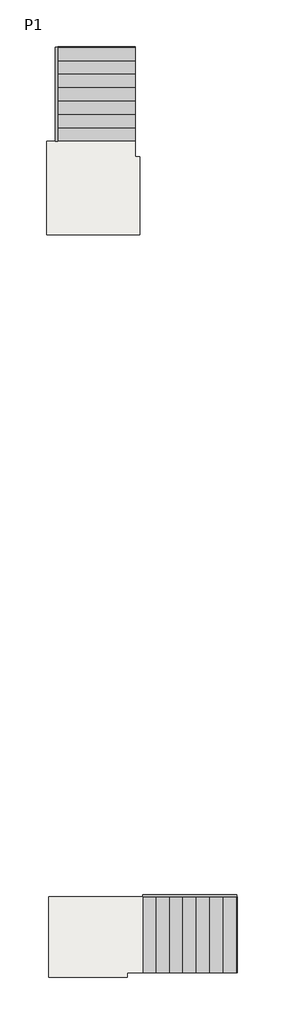
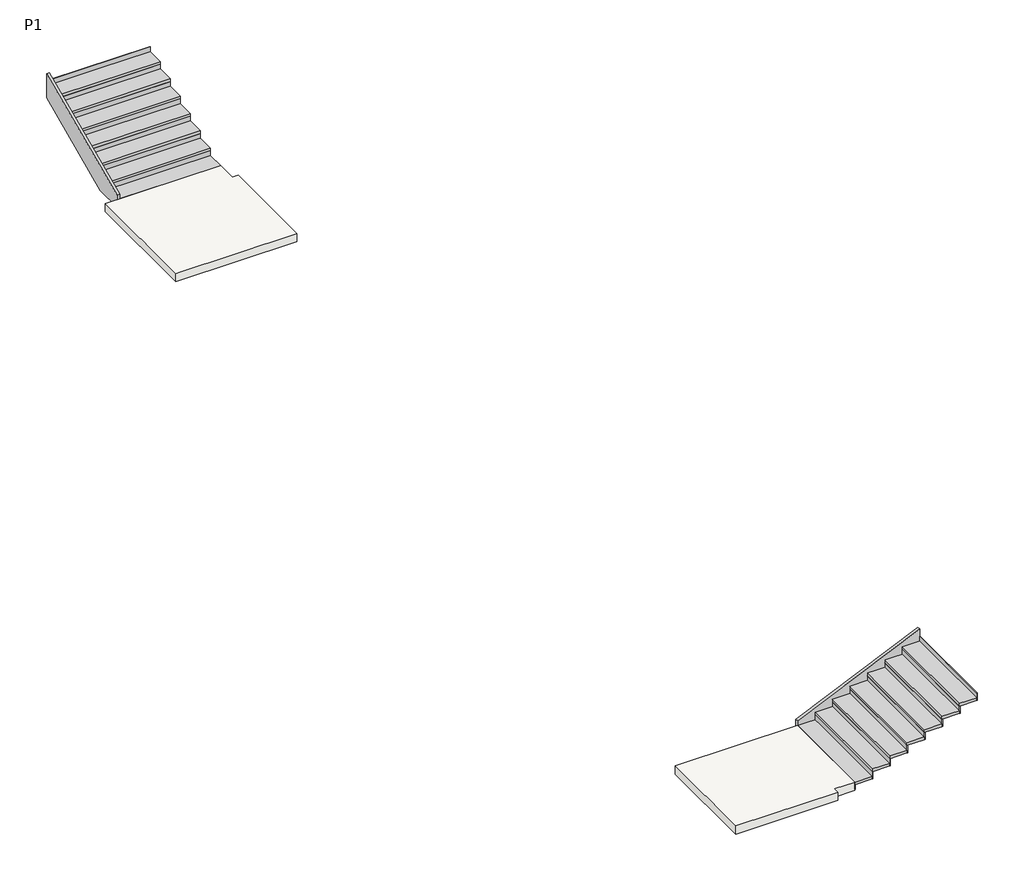
# One storey: 2 members, 2 slabs, 2 stair flights.
"""IFC4 building model written with IfcOpenShell, lengths in millimetres."""

import ifcopenshell
import ifcopenshell.guid

model = None  # the IFC model being written
_history = None  # IfcOwnerHistory: only IFC2X3 demands one
_inside = {}  # id of a spatial element -> (the spatial element, [elements in it])
_under = {}  # id of a project, library or spatial element -> (it, [spatial elements below it])
_declared = {}  # id of a project -> (the project, [libraries it declares])
_typed = {}  # id of a type object -> (the type object, [elements of that type])
_made_of = {}  # id of a material, layer set ... -> (it, [elements and type objects made of it])


def new_model(schema):
    """Start an empty IFC model of exactly this schema.

    Asked for "IFC4X3", IfcOpenShell would pick the latest addendum, in which some entities
    have other attributes; the version numbers below select the first issue.
    IFC2X3 requires an IfcOwnerHistory on every rooted entity: one is made here for all.
    """
    global model, _history
    if schema == "IFC4X3":
        model = ifcopenshell.file(schema_version=(4, 3, 0, 0))
    else:
        model = ifcopenshell.file(schema=schema)
    _inside.clear()
    _under.clear()
    _declared.clear()
    _typed.clear()
    _made_of.clear()
    _history = None
    if model.schema == "IFC2X3":
        org = make("IfcOrganization", Name="unknown")
        user = make(
            "IfcPersonAndOrganization",
            ThePerson=make("IfcPerson", FamilyName="unknown"),
            TheOrganization=org,
        )
        app = make(
            "IfcApplication",
            ApplicationDeveloper=org,
            Version="unknown",
            ApplicationFullName="unknown",
            ApplicationIdentifier="unknown",
        )
        _history = make(
            "IfcOwnerHistory",
            OwningUser=user,
            OwningApplication=app,
            ChangeAction="ADDED",
            CreationDate=0,
        )
    return model


def make(cls, **values):
    """One entity of the class cls with the attributes given. An attribute that is None is left unset."""
    return model.create_entity(
        cls, **{name: value for name, value in values.items() if value is not None}
    )


def rooted(cls, **values):
    """An entity with a GlobalId (a new one), such as an element, a storey or a relation."""
    return make(cls, GlobalId=ifcopenshell.guid.new(), OwnerHistory=_history, **values)


def si_unit(unit_type, name, prefix=None):
    """IfcSIUnit, for example si_unit("LENGTHUNIT", "METRE", prefix="MILLI")."""
    return make("IfcSIUnit", UnitType=unit_type, Prefix=prefix, Name=name)


def assignment(units):
    """IfcUnitAssignment: the units of a project."""
    return None if units is None else make("IfcUnitAssignment", Units=units)


def point(xyz):
    """IfcCartesianPoint."""
    return None if xyz is None else make("IfcCartesianPoint", Coordinates=xyz)


def direction(xyz):
    """IfcDirection."""
    return None if xyz is None else make("IfcDirection", DirectionRatios=xyz)


def frame(location, z_axis=None, x_axis=None):
    """IfcAxis2Placement3D, a coordinate frame: its origin and axes. An axis left out is left unset."""
    return make(
        "IfcAxis2Placement3D",
        Location=point(location),
        Axis=direction(z_axis),
        RefDirection=direction(x_axis),
    )


def origin():
    """The frame at (0, 0, 0) with its axes left unset."""
    return frame((0.0, 0.0, 0.0))


def place(relative_to, where):
    """IfcLocalPlacement: puts the frame where relative to a parent placement (None: the world)."""
    return make(
        "IfcLocalPlacement", PlacementRelTo=relative_to, RelativePlacement=where
    )


def context(
    kind, dimensions, precision=None, world=None, true_north=None, identifier=None
):
    """IfcGeometricRepresentationContext, for example the 3D "Model" context."""
    return make(
        "IfcGeometricRepresentationContext",
        ContextIdentifier=identifier,
        ContextType=kind,
        CoordinateSpaceDimension=dimensions,
        Precision=precision,
        WorldCoordinateSystem=world,
        TrueNorth=true_north,
    )


def project(units=None, contexts=None):
    """IfcProject with its units and contexts."""
    return rooted(
        "IfcProject",
        Name="project",
        RepresentationContexts=contexts,
        UnitsInContext=assignment(units),
    )


def spatial(cls, under=None, at=None, **own):
    """A site, building, storey or space (cls), placed at a placement, below another one or the project."""
    s = rooted(cls, ObjectPlacement=at, **own)
    if under is not None:
        _under.setdefault(under.id(), (under, []))[1].append(s)
    return s


def polyline(points):
    """IfcPolyline through the points."""
    return make("IfcPolyline", Points=[point(p) for p in points])


def outline(outer, holes=None, kind="AREA"):
    """IfcArbitraryClosedProfileDef: a profile drawn as a closed curve; with holes, ...WithVoids."""
    if holes is None:
        return make("IfcArbitraryClosedProfileDef", ProfileType=kind, OuterCurve=outer)
    return make(
        "IfcArbitraryProfileDefWithVoids",
        ProfileType=kind,
        OuterCurve=outer,
        InnerCurves=holes,
    )


def extrude(swept, where, along, depth):
    """IfcExtrudedAreaSolid: the profile swept, set in the frame where, extruded along a direction by depth."""
    return make(
        "IfcExtrudedAreaSolid",
        SweptArea=swept,
        Position=where,
        ExtrudedDirection=direction(along),
        Depth=depth,
    )


def shape(context_of_items, identifier, shape_type, items):
    """IfcShapeRepresentation: the items that make up one representation, for example the "Body"."""
    return make(
        "IfcShapeRepresentation",
        ContextOfItems=context_of_items,
        RepresentationIdentifier=identifier,
        RepresentationType=shape_type,
        Items=items,
    )


def source(mapping_origin, context_of_items, identifier, shape_type, items):
    """IfcRepresentationMap: a shape defined once, which mapped items show again and again."""
    return make(
        "IfcRepresentationMap",
        MappingOrigin=mapping_origin,
        MappedRepresentation=shape(context_of_items, identifier, shape_type, items),
    )


def transform(
    local_origin,
    x_axis=None,
    y_axis=None,
    z_axis=None,
    scale=None,
    scale2=None,
    scale3=None,
    uniform=True,
):
    """IfcCartesianTransformationOperator3D, or its non-uniform kind. x_axis, y_axis, z_axis: its Axis1, 2, 3."""
    if uniform:
        return make(
            "IfcCartesianTransformationOperator3D",
            Axis1=direction(x_axis),
            Axis2=direction(y_axis),
            LocalOrigin=point(local_origin),
            Scale=scale,
            Axis3=direction(z_axis),
        )
    return make(
        "IfcCartesianTransformationOperator3DnonUniform",
        Axis1=direction(x_axis),
        Axis2=direction(y_axis),
        LocalOrigin=point(local_origin),
        Scale=scale,
        Axis3=direction(z_axis),
        Scale2=scale2,
        Scale3=scale3,
    )


def mapped(mapping_source, mapping_target):
    """IfcMappedItem: shows the shape of a source again, moved by a transform."""
    return make(
        "IfcMappedItem", MappingSource=mapping_source, MappingTarget=mapping_target
    )


def made_of(thing, what):
    """Note that an element or type object is made of a material, layer set ...; save() writes the relation."""
    if what is not None:
        _made_of.setdefault(what.id(), (what, []))[1].append(thing)
    return thing


def element(
    cls,
    number,
    at=None,
    inside=None,
    cuts=None,
    type_object=None,
    material=None,
    context=None,
    identifier="Body",
    shape_type=None,
    held_by="IfcProductDefinitionShape",
    body=None,
    shapes=None,
    **own,
):
    """One element of the class cls, such as IfcWall. Its Tag is "e" and its number.

    at: its placement. inside: the storey or other place that contains it. cuts: it is an
    opening in that element (IfcRelVoidsElement). A single representation is given by context,
    identifier, shape_type and body (its items); several are given by shapes. held_by: the class
    of the entity that holds the representations. save() writes the other relations.
    """
    e = rooted(cls, Tag="e%d" % number, ObjectPlacement=at, **own)
    if body is not None:
        shapes = [shape(context, identifier, shape_type, body)]
    if shapes is not None:
        e.Representation = make(held_by, Representations=shapes)
    if inside is not None:
        _inside.setdefault(inside.id(), (inside, []))[1].append(e)
    if cuts is not None:
        rooted(
            "IfcRelVoidsElement", RelatingBuildingElement=cuts, RelatedOpeningElement=e
        )
    if type_object is not None:
        _typed.setdefault(type_object.id(), (type_object, []))[1].append(e)
    return made_of(e, material)


def aggregate(whole, parts):
    """IfcRelAggregates: a whole, such as a stair, and the parts it consists of."""
    return rooted("IfcRelAggregates", RelatingObject=whole, RelatedObjects=parts)


def save(model, path):
    """Write the relations noted so far, then the file.

    IfcRelAggregates (storeys below a building ...), IfcRelContainedInSpatialStructure (elements
    in a storey), IfcRelDefinesByType, IfcRelAssociatesMaterial and IfcRelDeclares: one each for
    every whole, place, type object, material and project.
    """
    for whole, parts in _under.values():
        aggregate(whole, parts)
    for where, things in _inside.values():
        rooted(
            "IfcRelContainedInSpatialStructure",
            RelatedElements=things,
            RelatingStructure=where,
        )
    for kind, things in _typed.values():
        rooted("IfcRelDefinesByType", RelatedObjects=things, RelatingType=kind)
    for what, things in _made_of.values():
        rooted("IfcRelAssociatesMaterial", RelatedObjects=things, RelatingMaterial=what)
    for by, libraries in _declared.values():
        rooted("IfcRelDeclares", RelatingContext=by, RelatedDefinitions=libraries)
    model.write(path)


def stair_flight_50mm_tread_13mm_riser_0aac887c(model_context):
    return source(origin(), model_context, "Body", "SweptSolid", [
        extrude(outline(polyline([(-15644.418089, 13093.1768963), (-15644.418089, 13080.6768963), (-17374.418089, 13080.6768963), (-17374.418089, 13093.1768963), (-15644.418089, 13093.1768963)])), frame((0.0, 0.0, -2133.3333333), z_axis=(0.0, 0.0, 1.0), x_axis=(1.0, 0.0, 0.0)), (0.0, 0.0, 1.0), 83.3333333),
        extrude(outline(polyline([(-17374.418089, 13380.6768963), (-15644.418089, 13380.6768963), (-15644.418089, 13080.6768963), (-17374.418089, 13080.6768963), (-17374.418089, 13380.6768963)])), frame((0.0, 0.0, -2050.0), z_axis=(0.0, 0.0, 1.0), x_axis=(1.0, 0.0, 0.0)), (0.0, 0.0, 1.0), 50.0),
        extrude(outline(polyline([(-15644.418089, 13393.1768963), (-15644.418089, 13380.6768963), (-17374.418089, 13380.6768963), (-17374.418089, 13393.1768963), (-15644.418089, 13393.1768963)])), frame((0.0, 0.0, -2050.0), z_axis=(0.0, 0.0, 1.0), x_axis=(1.0, 0.0, 0.0)), (0.0, 0.0, 1.0), 133.3333333),
        extrude(outline(polyline([(-17374.418089, 13680.6768963), (-15644.418089, 13680.6768963), (-15644.418089, 13380.6768963), (-17374.418089, 13380.6768963), (-17374.418089, 13680.6768963)])), frame((0.0, 0.0, -1916.6666667), z_axis=(0.0, 0.0, 1.0), x_axis=(1.0, 0.0, 0.0)), (0.0, 0.0, 1.0), 50.0),
        extrude(outline(polyline([(-15644.418089, 13693.1768963), (-15644.418089, 13680.6768963), (-17374.418089, 13680.6768963), (-17374.418089, 13693.1768963), (-15644.418089, 13693.1768963)])), frame((0.0, 0.0, -1916.6666667), z_axis=(0.0, 0.0, 1.0), x_axis=(1.0, 0.0, 0.0)), (0.0, 0.0, 1.0), 133.3333333),
        extrude(outline(polyline([(-17374.418089, 13980.6768963), (-15644.418089, 13980.6768963), (-15644.418089, 13680.6768963), (-17374.418089, 13680.6768963), (-17374.418089, 13980.6768963)])), frame((0.0, 0.0, -1783.3333333), z_axis=(0.0, 0.0, 1.0), x_axis=(1.0, 0.0, 0.0)), (0.0, 0.0, 1.0), 50.0),
        extrude(outline(polyline([(-15644.418089, 13993.1768963), (-15644.418089, 13980.6768963), (-17374.418089, 13980.6768963), (-17374.418089, 13993.1768963), (-15644.418089, 13993.1768963)])), frame((0.0, 0.0, -1783.3333333), z_axis=(0.0, 0.0, 1.0), x_axis=(1.0, 0.0, 0.0)), (0.0, 0.0, 1.0), 133.3333333),
        extrude(outline(polyline([(-17374.418089, 14280.6768963), (-15644.418089, 14280.6768963), (-15644.418089, 13980.6768963), (-17374.418089, 13980.6768963), (-17374.418089, 14280.6768963)])), frame((0.0, 0.0, -1650.0), z_axis=(0.0, 0.0, 1.0), x_axis=(1.0, 0.0, 0.0)), (0.0, 0.0, 1.0), 50.0),
        extrude(outline(polyline([(-15644.418089, 14293.1768963), (-15644.418089, 14280.6768963), (-17374.418089, 14280.6768963), (-17374.418089, 14293.1768963), (-15644.418089, 14293.1768963)])), frame((0.0, 0.0, -1650.0), z_axis=(0.0, 0.0, 1.0), x_axis=(1.0, 0.0, 0.0)), (0.0, 0.0, 1.0), 133.3333333),
        extrude(outline(polyline([(-17374.418089, 14580.6768963), (-15644.418089, 14580.6768963), (-15644.418089, 14280.6768963), (-17374.418089, 14280.6768963), (-17374.418089, 14580.6768963)])), frame((0.0, 0.0, -1516.6666667), z_axis=(0.0, 0.0, 1.0), x_axis=(1.0, 0.0, 0.0)), (0.0, 0.0, 1.0), 50.0),
        extrude(outline(polyline([(-15644.418089, 14593.1768963), (-15644.418089, 14580.6768963), (-17374.418089, 14580.6768963), (-17374.418089, 14593.1768963), (-15644.418089, 14593.1768963)])), frame((0.0, 0.0, -1516.6666667), z_axis=(0.0, 0.0, 1.0), x_axis=(1.0, 0.0, 0.0)), (0.0, 0.0, 1.0), 133.3333333),
        extrude(outline(polyline([(-17374.418089, 14880.6768963), (-15644.418089, 14880.6768963), (-15644.418089, 14580.6768963), (-17374.418089, 14580.6768963), (-17374.418089, 14880.6768963)])), frame((0.0, 0.0, -1383.3333333), z_axis=(0.0, 0.0, 1.0), x_axis=(1.0, 0.0, 0.0)), (0.0, 0.0, 1.0), 50.0),
        extrude(outline(polyline([(-15644.418089, 14893.1768963), (-15644.418089, 14880.6768963), (-17374.418089, 14880.6768963), (-17374.418089, 14893.1768963), (-15644.418089, 14893.1768963)])), frame((0.0, 0.0, -1383.3333333), z_axis=(0.0, 0.0, 1.0), x_axis=(1.0, 0.0, 0.0)), (0.0, 0.0, 1.0), 133.3333333),
        extrude(outline(polyline([(-15644.418089, 15193.1768963), (-15644.418089, 15180.6768963), (-17374.418089, 15180.6768963), (-17374.418089, 15193.1768963), (-15644.418089, 15193.1768963)])), frame((0.0, 0.0, -1250.0), z_axis=(0.0, 0.0, 1.0), x_axis=(1.0, 0.0, 0.0)), (0.0, 0.0, 1.0), 133.3333333),
        extrude(outline(polyline([(-17374.418089, 15180.6768963), (-15644.418089, 15180.6768963), (-15644.418089, 14880.6768963), (-17374.418089, 14880.6768963), (-17374.418089, 15180.6768963)])), frame((0.0, 0.0, -1250.0), z_axis=(0.0, 0.0, 1.0), x_axis=(1.0, 0.0, 0.0)), (0.0, 0.0, 1.0), 50.0),
    ])


def stair_flight_50mm_tread_13mm_riser_cbb1d095(model_context):
    return source(origin(), model_context, "Body", "SweptSolid", [
        extrude(outline(polyline([(-15462.7814495, -5518.0731037), (-15475.2814495, -5518.0731037), (-15475.2814495, -3818.0731037), (-15462.7814495, -3818.0731037), (-15462.7814495, -5518.0731037)])), frame((0.0, 0.0, -2133.3333333), z_axis=(0.0, 0.0, 1.0), x_axis=(1.0, 0.0, 0.0)), (0.0, 0.0, 1.0), 83.3333333),
        extrude(outline(polyline([(-15175.2814495, -3818.0731037), (-15175.2814495, -5518.0731037), (-15475.2814495, -5518.0731037), (-15475.2814495, -3818.0731037), (-15175.2814495, -3818.0731037)])), frame((0.0, 0.0, -2050.0), z_axis=(0.0, 0.0, 1.0), x_axis=(1.0, 0.0, 0.0)), (0.0, 0.0, 1.0), 50.0),
        extrude(outline(polyline([(-15162.7814495, -5518.0731037), (-15175.2814495, -5518.0731037), (-15175.2814495, -3818.0731037), (-15162.7814495, -3818.0731037), (-15162.7814495, -5518.0731037)])), frame((0.0, 0.0, -2050.0), z_axis=(0.0, 0.0, 1.0), x_axis=(1.0, 0.0, 0.0)), (0.0, 0.0, 1.0), 133.3333333),
        extrude(outline(polyline([(-14875.2814495, -3818.0731037), (-14875.2814495, -5518.0731037), (-15175.2814495, -5518.0731037), (-15175.2814495, -3818.0731037), (-14875.2814495, -3818.0731037)])), frame((0.0, 0.0, -1916.6666667), z_axis=(0.0, 0.0, 1.0), x_axis=(1.0, 0.0, 0.0)), (0.0, 0.0, 1.0), 50.0),
        extrude(outline(polyline([(-14862.7814495, -5518.0731037), (-14875.2814495, -5518.0731037), (-14875.2814495, -3818.0731037), (-14862.7814495, -3818.0731037), (-14862.7814495, -5518.0731037)])), frame((0.0, 0.0, -1916.6666667), z_axis=(0.0, 0.0, 1.0), x_axis=(1.0, 0.0, 0.0)), (0.0, 0.0, 1.0), 133.3333333),
        extrude(outline(polyline([(-14575.2814495, -3818.0731037), (-14575.2814495, -5518.0731037), (-14875.2814495, -5518.0731037), (-14875.2814495, -3818.0731037), (-14575.2814495, -3818.0731037)])), frame((0.0, 0.0, -1783.3333333), z_axis=(0.0, 0.0, 1.0), x_axis=(1.0, 0.0, 0.0)), (0.0, 0.0, 1.0), 50.0),
        extrude(outline(polyline([(-14562.7814495, -5518.0731037), (-14575.2814495, -5518.0731037), (-14575.2814495, -3818.0731037), (-14562.7814495, -3818.0731037), (-14562.7814495, -5518.0731037)])), frame((0.0, 0.0, -1783.3333333), z_axis=(0.0, 0.0, 1.0), x_axis=(1.0, 0.0, 0.0)), (0.0, 0.0, 1.0), 133.3333333),
        extrude(outline(polyline([(-14275.2814495, -3818.0731037), (-14275.2814495, -5518.0731037), (-14575.2814495, -5518.0731037), (-14575.2814495, -3818.0731037), (-14275.2814495, -3818.0731037)])), frame((0.0, 0.0, -1650.0), z_axis=(0.0, 0.0, 1.0), x_axis=(1.0, 0.0, 0.0)), (0.0, 0.0, 1.0), 50.0),
        extrude(outline(polyline([(-14262.7814495, -5518.0731037), (-14275.2814495, -5518.0731037), (-14275.2814495, -3818.0731037), (-14262.7814495, -3818.0731037), (-14262.7814495, -5518.0731037)])), frame((0.0, 0.0, -1650.0), z_axis=(0.0, 0.0, 1.0), x_axis=(1.0, 0.0, 0.0)), (0.0, 0.0, 1.0), 133.3333333),
        extrude(outline(polyline([(-13975.2814495, -3818.0731037), (-13975.2814495, -5518.0731037), (-14275.2814495, -5518.0731037), (-14275.2814495, -3818.0731037), (-13975.2814495, -3818.0731037)])), frame((0.0, 0.0, -1516.6666667), z_axis=(0.0, 0.0, 1.0), x_axis=(1.0, 0.0, 0.0)), (0.0, 0.0, 1.0), 50.0),
        extrude(outline(polyline([(-13962.7814495, -5518.0731037), (-13975.2814495, -5518.0731037), (-13975.2814495, -3818.0731037), (-13962.7814495, -3818.0731037), (-13962.7814495, -5518.0731037)])), frame((0.0, 0.0, -1516.6666667), z_axis=(0.0, 0.0, 1.0), x_axis=(1.0, 0.0, 0.0)), (0.0, 0.0, 1.0), 133.3333333),
        extrude(outline(polyline([(-13675.2814495, -3818.0731037), (-13675.2814495, -5518.0731037), (-13975.2814495, -5518.0731037), (-13975.2814495, -3818.0731037), (-13675.2814495, -3818.0731037)])), frame((0.0, 0.0, -1383.3333333), z_axis=(0.0, 0.0, 1.0), x_axis=(1.0, 0.0, 0.0)), (0.0, 0.0, 1.0), 50.0),
        extrude(outline(polyline([(-13662.7814495, -5518.0731037), (-13675.2814495, -5518.0731037), (-13675.2814495, -3818.0731037), (-13662.7814495, -3818.0731037), (-13662.7814495, -5518.0731037)])), frame((0.0, 0.0, -1383.3333333), z_axis=(0.0, 0.0, 1.0), x_axis=(1.0, 0.0, 0.0)), (0.0, 0.0, 1.0), 133.3333333),
        extrude(outline(polyline([(-13362.7814495, -5518.0731037), (-13375.2814495, -5518.0731037), (-13375.2814495, -3818.0731037), (-13362.7814495, -3818.0731037), (-13362.7814495, -5518.0731037)])), frame((0.0, 0.0, -1250.0), z_axis=(0.0, 0.0, 1.0), x_axis=(1.0, 0.0, 0.0)), (0.0, 0.0, 1.0), 133.3333333),
        extrude(outline(polyline([(-13375.2814495, -3818.0731037), (-13375.2814495, -5518.0731037), (-13675.2814495, -5518.0731037), (-13675.2814495, -3818.0731037), (-13375.2814495, -3818.0731037)])), frame((0.0, 0.0, -1250.0), z_axis=(0.0, 0.0, 1.0), x_axis=(1.0, 0.0, 0.0)), (0.0, 0.0, 1.0), 50.0),
    ])


model = new_model("IFC4")

# Units and contexts
model_context = context("Model", 3, world=origin())
ifc_project = project(units=[si_unit("LENGTHUNIT", "METRE", prefix="MILLI")], contexts=[model_context])

# Site, building, storey
site = spatial("IfcSite", under=ifc_project)
building = spatial("IfcBuilding", under=site)
storey = spatial("IfcBuildingStorey", under=building, Name="P1", Elevation=-2133.3333333)

# Members
placement = place(None, origin())
element("IfcMember", 1, ObjectType="Stringer - 50mm Width", at=placement, inside=storey, context=model_context, shape_type="SweptSolid", body=[
    extrude(outline(polyline([(13080.6768963, -2133.3333333), (13080.6768963, -1915.3095055), (15180.6768963, -981.9761722), (15180.6768963, -1419.7031856), (13575.0090639, -2133.3333333), (13080.6768963, -2133.3333333)])), frame((-17424.418089, 0.0, 0.0), z_axis=(1.0, 0.0, 0.0), x_axis=(0.0, 1.0, 0.0)), (0.0, 0.0, 1.0), 50.0),
])
element("IfcMember", 2, ObjectType="Stringer - 50mm Width", at=placement, inside=storey, context=model_context, shape_type="SweptSolid", body=[
    extrude(outline(polyline([(-1915.3095055, -15475.2814495), (-2133.3333333, -15475.2814495), (-2133.3333333, -14980.9492819), (-1419.7031856, -13375.2814495), (-981.9761722, -13375.2814495), (-1915.3095055, -15475.2814495)])), frame((0.0, -3818.0731037, 0.0), z_axis=(0.0, 1.0, 0.0), x_axis=(0.0, 0.0, 1.0)), (0.0, 0.0, 1.0), 50.0),
])

# Slabs
element("IfcSlab", 3, ObjectType="Generic 150mm", at=placement, inside=storey, context=model_context, shape_type="SweptSolid", body=[
    extrude(outline(polyline([(-15644.418089, 12730.6768963), (-15544.418089, 12730.6768963), (-15544.418089, 10980.6768963), (-17624.418089, 10980.6768963), (-17624.418089, 13080.6768963), (-15644.418089, 13080.6768963), (-15644.418089, 12730.6768963)])), frame((0.0, 0.0, -2150.0), z_axis=(0.0, 0.0, 1.0), x_axis=(1.0, 0.0, 0.0)), (0.0, 0.0, 1.0), 150.0),
])
element("IfcSlab", 4, ObjectType="Generic 150mm", at=placement, inside=storey, context=model_context, shape_type="SweptSolid", body=[
    extrude(outline(polyline([(-15825.2814495, -5518.0731037), (-15825.2814495, -5618.0731037), (-17575.2814495, -5618.0731037), (-17575.2814495, -3818.0731037), (-15475.2814495, -3818.0731037), (-15475.2814495, -5518.0731037), (-15825.2814495, -5518.0731037)])), frame((0.0, 0.0, -2150.0), z_axis=(0.0, 0.0, 1.0), x_axis=(1.0, 0.0, 0.0)), (0.0, 0.0, 1.0), 150.0),
])

# Stair flights
stair_flight_50mm_tread_13mm_riser_shape = stair_flight_50mm_tread_13mm_riser_0aac887c(model_context)
element("IfcStairFlight", 5, ObjectType="50mm Tread 13mm Riser", at=placement, inside=storey, context=model_context, shape_type="MappedRepresentation", body=[
    mapped(stair_flight_50mm_tread_13mm_riser_shape, transform((0.0, 0.0, 0.0), x_axis=(1.0, 0.0, 0.0), y_axis=(0.0, 1.0, 0.0), z_axis=(0.0, 0.0, 1.0))),
])
stair_flight_50mm_tread_13mm_riser_2_shape = stair_flight_50mm_tread_13mm_riser_cbb1d095(model_context)
element("IfcStairFlight", 6, ObjectType="50mm Tread 13mm Riser", at=placement, inside=storey, context=model_context, shape_type="MappedRepresentation", body=[
    mapped(stair_flight_50mm_tread_13mm_riser_2_shape, transform((0.0, 0.0, 0.0), x_axis=(1.0, 0.0, 0.0), y_axis=(0.0, 1.0, 0.0), z_axis=(0.0, 0.0, 1.0))),
])

save(model, "model.ifc")

# Revit data of these elements
# Type "Generic 150mm"
#   Function = 0
#   Layers, outside or top first: 15 cm no material (function 1)
# Elements 1, 2 (IfcMember, "Stringer - 50mm Width")
#   Phase Created = New Construction
# Element 3 (IfcSlab, "Generic 150mm")
#   built-in parameter 1001955 = -1.5708 (stored number, unit not read)
#   Height Offset From Level = 13.3333 cm
#   Phase Created = New Construction
#   Materials on its faces: "Default Floor"
# Element 4 (IfcSlab, "Generic 150mm")
#   built-in parameter 1001955 = -3.14159 (stored number, unit not read)
#   Height Offset From Level = 13.3333 cm
#   Phase Created = New Construction
#   Materials on its faces: "Default Floor"
# Elements 5, 6 (IfcStairFlight, "50mm Tread 13mm Riser")
#   Phase Created = New Construction
# Materials
#   "Default Floor": class "Miscellaneous", colour RGB 127 127 127, transparency 0, Cost = 0
